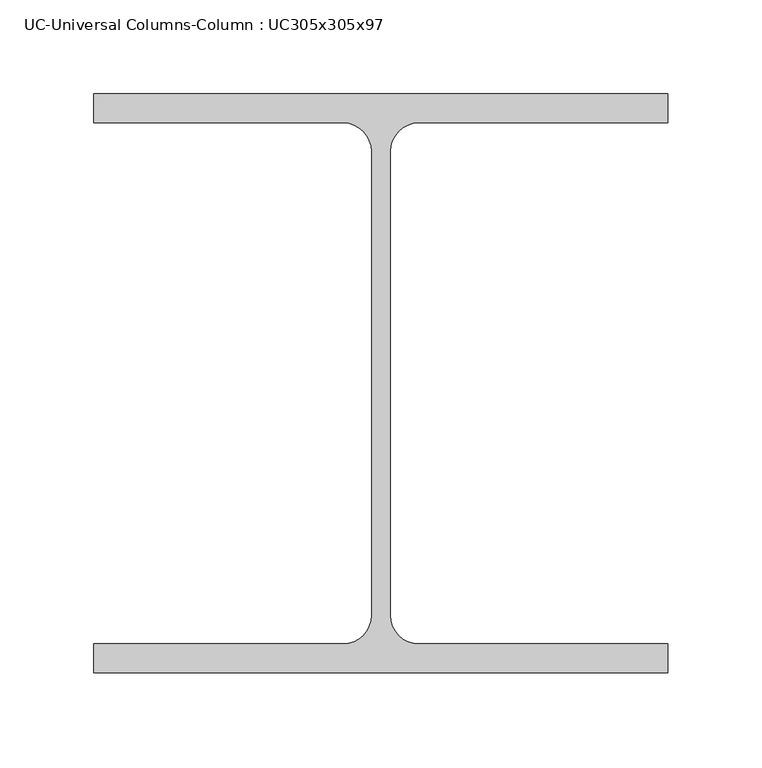
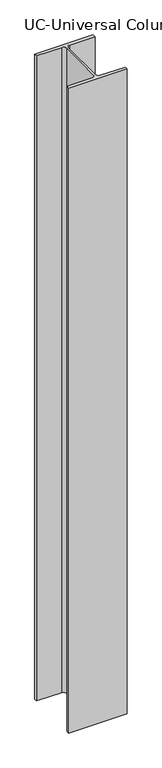
"""IFC4 building model written with IfcOpenShell, lengths in millimetres: column geometry, UC-Universal Columns-Column : UC305x305x97."""

from ifc_helpers import new_model, si_unit, point, frame, frame_2d, origin, place, context, project, spatial, polyline, circle_curve, trimmed, segment, composite_curve, outline, extrude, source, transform, mapped, element, save


def uc_universal_columns_column_uc305x305x97_d52c2ea7(model_context):
    return source(origin(), model_context, "Body", "SweptSolid", [
        extrude(outline(composite_curve([segment(polyline([(152.65, 153.95), (152.65, 138.55), (20.15, 138.55)]), True, "CONTINUOUS"), segment(trimmed(circle_curve(frame_2d((20.15, 123.35)), 15.2), [point((20.15, 138.55))], [point((4.95, 123.35))], True, "CARTESIAN"), True, "CONTINUOUS"), segment(polyline([(4.95, 123.35), (4.95, -123.35)]), True, "CONTINUOUS"), segment(trimmed(circle_curve(frame_2d((20.15, -123.35)), 15.2), [point((4.95, -123.35))], [point((20.15, -138.55))], True, "CARTESIAN"), True, "CONTINUOUS"), segment(polyline([(20.15, -138.55), (152.65, -138.55), (152.65, -153.95), (-152.65, -153.95), (-152.65, -138.55), (-20.15, -138.55)]), True, "CONTINUOUS"), segment(trimmed(circle_curve(frame_2d((-20.15, -123.35)), 15.2), [point((-20.15, -138.55))], [point((-4.95, -123.35))], True, "CARTESIAN"), True, "CONTINUOUS"), segment(polyline([(-4.95, -123.35), (-4.95, 123.35)]), True, "CONTINUOUS"), segment(trimmed(circle_curve(frame_2d((-20.15, 123.35)), 15.2), [point((-4.95, 123.35))], [point((-20.15, 138.55))], True, "CARTESIAN"), True, "CONTINUOUS"), segment(polyline([(-20.15, 138.55), (-152.65, 138.55), (-152.65, 153.95), (152.65, 153.95)]), True, "CONTINUOUS")], self_intersect=False)), frame((0.0, 0.0, 2439.0), z_axis=(0.0, 0.0, 1.0), x_axis=(1.0, 0.0, 0.0)), (0.0, 0.0, 1.0), 3561.0),
    ])


if __name__ == "__main__":
    model = new_model("IFC4")
    model_context = context("Model", 3, world=origin())
    ifc_project = project(units=[si_unit("LENGTHUNIT", "METRE", prefix="MILLI")], contexts=[model_context])
    site = spatial("IfcSite", under=ifc_project)
    building = spatial("IfcBuilding", under=site)
    placement = place(None, origin())
    uc_universal_columns_column_uc305x305x97_shape = uc_universal_columns_column_uc305x305x97_d52c2ea7(model_context)
    element("IfcColumn", 1, ObjectType="UC-Universal Columns-Column : UC305x305x97", at=placement, inside=building, context=model_context, shape_type="MappedRepresentation", body=[
        mapped(uc_universal_columns_column_uc305x305x97_shape, transform((0.0, 0.0, 0.0), x_axis=(1.0, 0.0, 0.0), y_axis=(0.0, 1.0, 0.0), z_axis=(0.0, 0.0, 1.0))),
    ])
    save(model, "model.ifc")

# Revit data of these elements
# Type "UC-Universal Columns-Column : UC305x305x97"
#   Section Name Key = "UC305x305x97"
#   Cost = 2
#   Width = 30.53 cm
#   Web Thickness = 0.99 cm
#   Web Fillet = 1.52 cm
#   Warping Constant = 1560000.0 cm⁶
#   Torsional Moment of Inertia = 91.20 cm⁴
#   Section Area = 123.0 cm²
#   Plastic Modulus weak axis = 726.0 cm³
#   Plastic Modulus strong axis = 1592.0 cm³
#   Nominal Weight = 96.8996 kgf/m
#   Moment of Inertia weak axis = 7308.00 cm⁴
#   Moment of Inertia strong axis = 22249.00 cm⁴
#   Height = 30.79 cm
#   Flange Thickness = 1.54 cm
#   Elastic Modulus weak axis = 479.0 cm³
#   Elastic Modulus strong axis = 1445.0 cm³
#   Centroid Vertical = 15.395 cm
#   Centroid Horizontal = 15.265 cm
#   Bolt Spacing = 14.0 cm
#   Structural Material [instance default] = Metal - Steel 43-275
#   Type Comments = ""
#   Assembly Code = ""
# Element 1 (IfcColumn, "UC-Universal Columns-Column : UC305x305x97")
#   Materials on its faces: "Metal - Steel 43-275"
# Materials
#   "Metal - Steel 43-275": class "Metal", colour RGB 247 247 247, transparency 0, Cost = 0
